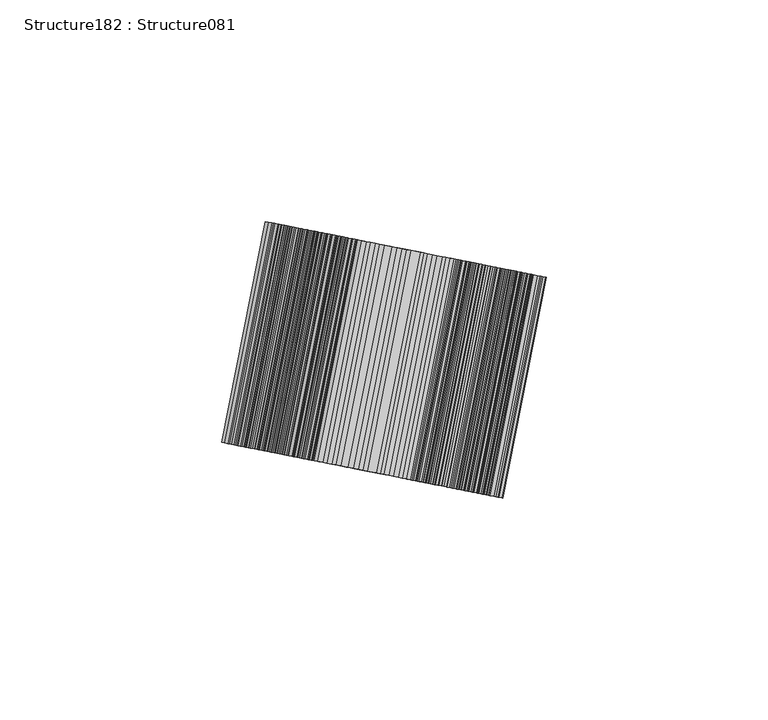
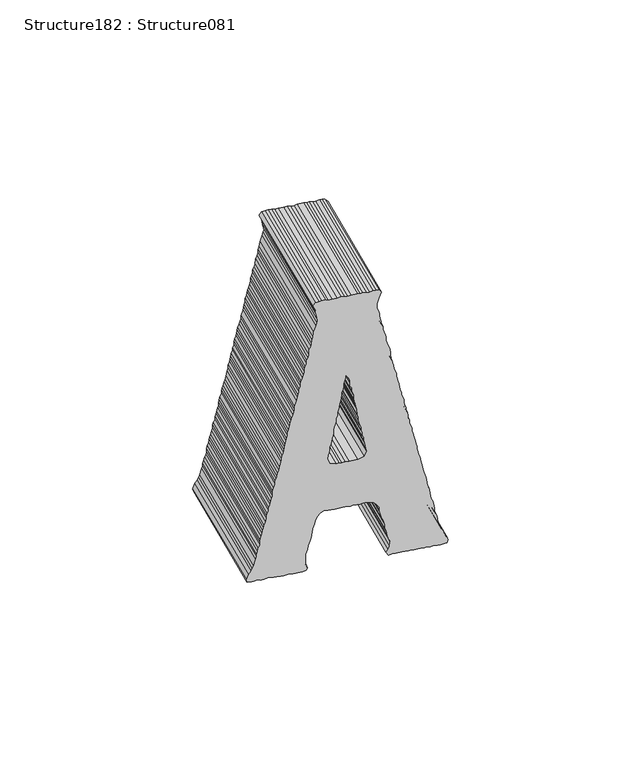
"""IFC4 building model written with IfcOpenShell, lengths in millimetres: proxy geometry, Structure182 : Structure081."""

from ifc_helpers import new_model, si_unit, frame, origin, place, context, project, spatial, polyline, outline, extrude, source, transform, mapped, element, save


def structure182_structure081_149fff3d(model_context):
    return source(origin(), model_context, "Body", "SweptSolid", [
        extrude(outline(polyline([(0.9094651, 0.0), (2.0811665, -0.5212701), (2.9906316, -0.6507871), (4.1562841, -0.780304), (5.1991801, -1.1720571), (5.9748585, -1.3012184), (7.1504738, -1.6890575), (8.1894559, -1.6890575), (9.3551083, -2.0808107), (10.2645735, -2.3398445), (11.4362748, -2.5981668), (12.3453841, -2.8611147), (13.3818755, -2.9902758), (14.1582655, -3.378115), (15.4626861, -3.509411), (16.3721513, -3.509411), (17.5385154, -3.7698682), (19.491944, -4.4188761), (20.2718921, -4.6793333), (21.3101626, -4.9383672), (22.3470097, -4.9383672), (23.2561191, -5.1988244), (24.4278204, -5.5866635), (25.4700048, -5.9766376), (26.6363689, -5.9766376), (27.4124031, -6.3666117), (28.7175354, -6.6274247), (30.535754, -7.0173988), (31.5743802, -7.1483389), (32.7400327, -7.4073728), (33.6555467, -7.7969911), (35.4741211, -7.7969911), (36.5102567, -7.5361781), (37.5492387, -7.275721), (38.3288311, -6.8878819), (39.3671015, -6.3666117), (40.4099976, -7.275721), (40.5395145, -8.1851861), (40.5395145, -9.0964303), (40.2826155, -10.2659967), (40.2826155, -11.3042672), (40.5395145, -12.4745453), (40.4099976, -13.2523586), (40.5395145, -14.1639585), (40.5395145, -16.2429902), (40.2826155, -17.2791257), (40.2826155, -18.3198869), (40.5395145, -19.4915882), (40.4099976, -20.6575964), (40.4099976, -22.3466539), (40.2826155, -23.5183553), (40.5395145, -24.4274646), (40.5395145, -25.595252), (40.4099976, -26.5047171), (40.2826155, -27.6742836), (39.2382962, -28.4545875), (38.3288311, -27.9372314), (37.4197218, -27.6742836), (36.6397736, -27.5454783), (35.4741211, -27.2846653), (33.5199809, -26.8964703), (32.6112274, -27.1576391), (31.4448633, -27.4138264), (29.3636968, -28.1937746), (27.545834, -28.4545875), (26.5089869, -28.7150447), (25.3372855, -28.8445616), (24.2943895, -29.1032397), (23.2561191, -29.6262889), (21.3101626, -29.7540268), (20.2718921, -30.0144839), (19.491944, -30.5336191), (18.3202426, -30.5336191), (17.2816164, -30.9235932), (16.3721513, -31.1840503), (15.3356599, -31.1840503), (14.1582655, -31.4427285), (13.1253323, -31.8330584), (12.2158672, -32.2230324), (11.4362748, -32.3518377), (10.2645735, -32.4834896), (9.3551083, -32.8731078), (8.1894559, -32.8731078), (7.1504738, -33.2613029), (6.2374505, -33.3925989), (5.0714422, -33.653056), (3.2475306, -34.302064), (2.0811665, -34.302064), (1.1720572, -34.5625212), (0.1334309, -34.8208434), (-1.0382704, -35.3421135), (-1.8178628, -35.4716305), (-2.8568449, -35.7303085), (-3.8990293, -35.8616046), (-5.0653934, -36.2515787), (-5.8471206, -36.5099009), (-7.0166871, -36.5099009), (-8.1826954, -36.899875), (-8.9644226, -37.0315268), (-10.1364798, -37.419366), (-11.1690572, -37.5506621), (-12.2115974, -37.680179), (-12.9915456, -37.9406362), (-14.03373, -38.3284753), (-15.3292552, -38.4601271), (-16.3678815, -38.7205843), (-18.1861001, -39.1084235), (-19.3581573, -39.3692365), (-20.2672666, -39.7574314), (-21.4371888, -40.0178886), (-22.2189161, -40.2783458), (-23.1223323, -40.5370239), (-24.1648726, -40.5370239), (-25.465735, -41.0586498), (-26.5025822, -41.316972), (-27.4173846, -41.4464889), (-28.4560108, -41.4464889), (-29.235959, -41.7069461), (-30.5311284, -42.0986993), (-31.3110766, -42.2264372), (-32.3536168, -42.6181903), (-33.5214042, -42.6181903), (-34.4308693, -43.1355464), (-35.3399786, -43.3960036), (-36.37647, -43.3960036), (-37.5424783, -43.6564608), (-38.7202285, -44.0442999), (-39.6236447, -44.3072478), (-40.405372, -44.5659258), (-41.5752942, -44.695087), (-42.6139205, -45.0850611), (-43.7856218, -45.3455183), (-44.8221132, -45.3455183), (-45.7372714, -45.4732561), (-46.6406876, -45.9963053), (-47.812389, -46.2549833), (-48.8510152, -46.5140173), (-49.7601245, -46.5140173), (-50.6731478, -46.9057704), (-52.8777823, -47.5540667), (-53.7929405, -47.941906), (-54.5689747, -48.3340149), (-55.738897, -49.1118282), (-57.5532016, -49.7626152), (-58.4665807, -49.5035814), (-58.5957419, -48.2030748), (-58.4665807, -47.4227707), (-58.3331498, -46.2549833), (-58.5957419, -45.2167129), (-58.5957419, -44.0442999), (-58.3331498, -43.0060295), (-58.3331498, -42.0986993), (-58.4665807, -41.0586498), (-58.4665807, -40.1491846), (-58.5957419, -38.8479664), (-58.5957419, -37.9406362), (-58.4665807, -36.899875), (-58.3331498, -35.7303085), (-58.5957419, -34.8208434), (-58.5957419, -31.8330584), (-58.3331498, -30.6627802), (-57.4297336, -30.1440009), (-56.6480063, -30.5336191), (-55.6115149, -30.7940763), (-53.3972734, -30.7940763), (-52.3586471, -30.7940763), (-51.4495378, -30.5336191), (-50.6731478, -30.1440009), (-49.3683714, -30.0144839), (-48.4592621, -29.7540268), (-47.5497969, -29.3636969), (-46.6406876, -29.1032397), (-45.6038405, -28.8445616), (-43.2661308, -28.5855278), (-41.5752942, -27.9372314), (-40.2762109, -27.6742836), (-38.9767716, -27.0259872), (-38.1950444, -26.116878), (-37.4190102, -24.6864985), (-37.6759092, -23.6478723), (-37.6759092, -21.5688406), (-37.5424783, -20.2694015), (-37.5424783, -17.5420735), (-37.6759092, -16.3700164), (-37.4190102, -15.463042), (-37.5424783, -14.4240599), (-37.6759092, -13.3840104), (-37.5424783, -12.4745453), (-37.4190102, -11.1754619), (-37.6759092, -10.3955138), (-38.0676623, -8.8373964), (-38.8476105, -8.0556692), (-40.2762109, -7.0173988), (-41.4422191, -7.0173988), (-42.6139205, -6.75623), (-44.561656, -6.2388738), (-45.3472973, -5.7179595), (-46.5133056, -5.4592815), (-47.2932538, -5.3283413), (-48.33188, -5.3283413), (-49.3683714, -4.8067153), (-50.4126907, -4.6793333), (-51.4495378, -4.5501722), (-52.3586471, -4.158419), (-53.6595096, -3.7698682), (-55.3489229, -3.897606), (-56.6480063, -4.2875802), (-57.2966585, -4.9383672), (-58.5957419, -4.158419), (-58.4665807, -2.9902758), (-58.3331498, -1.9498705), (-58.3331498, 0.1291611), (-58.4665807, 1.1677874), (-58.4665807, 2.2060577), (-58.3331498, 3.1176577), (-58.4665807, 4.0267671), (-58.4665807, 5.3258505), (-58.3331498, 6.1040195), (-58.4665807, 7.4052379), (-58.3331498, 8.1848303), (-58.5957419, 9.2252356), (-58.3331498, 10.3933787), (-58.5957419, 11.563301), (-58.4665807, 12.4724103), (-58.3331498, 13.5128156), (-58.3331498, 14.5496628), (-57.2966585, 14.941416), (-56.3875492, 14.6809589), (-55.738897, 14.0301718), (-54.5689747, 13.7718495), (-53.7929405, 13.3818755), (-52.6151903, 12.8602495), (-50.6731478, 11.9511402), (-49.8875066, 11.692818), (-48.5941162, 11.563301), (-47.5497969, 11.3028439), (-46.6406876, 11.04381), (-45.8646534, 10.6520569), (-44.5616561, 10.5225398), (-42.6139205, 10.2638618), (-41.4422191, 9.8738878), (-40.5384471, 9.4821345), (-39.6236447, 9.2252356), (-38.4576364, 9.0942954), (-37.4190102, 8.9626435), (-36.5059869, 8.8338382), (-35.6004358, 8.3143472), (-34.2956593, 8.1848303), (-33.3922431, 8.0535342), (-32.3536168, 7.9243731), (-31.4405935, 7.5365339), (-30.4019673, 7.1447807), (-29.235959, 6.8857468), (-27.5447666, 6.6252897), (-26.3752002, 6.2353156), (-25.203143, 6.1040195), (-24.4235506, 5.8474765), (-23.3849244, 5.4553674), (-22.4793732, 5.3258505), (-21.3037579, 4.9362323), (-20.2672666, 4.9362323), (-19.3581573, 4.6750634), (-18.319531, 4.4167412), (-17.1474738, 4.158419), (-15.2018732, 3.636793), (-14.1632469, 3.3777591), (-13.1207067, 3.3777591), (-12.2115974, 2.986006), (-11.3024881, 2.5981668), (-10.0012698, 2.5981668), (-9.2270147, 2.0772524), (-8.1826954, 2.0772524), (-7.0166871, 1.9498704), (-5.9745027, 1.4282444), (-5.0653934, 1.4282444), (-4.1619771, 0.9091093), (-2.8568449, 0.7799482), (-1.9473797, 0.7799482), (-0.7817273, 0.2604572), (0.0, 0.0), (0.9094651, 0.0)]), holes=[polyline([(-20.9137838, -13.9010107), (-20.9137838, -16.8912865), (-20.7903157, -18.0590739), (-21.0472147, -19.231131), (-20.7903157, -20.1398845), (-20.9137838, -21.0493497), (-20.2672666, -22.997441), (-18.5817672, -23.6478723), (-17.2809048, -23.3874152), (-16.3678815, -23.1262464), (-15.4623303, -22.870059), (-14.1632469, -22.997441), (-13.2480888, -22.47795), (-12.2115974, -22.3466539), (-11.3024881, -22.2174928), (-10.393023, -21.8292978), (-9.3508386, -21.6983577), (-8.3122123, -21.6983577), (-7.146204, -21.5688406), (-6.3644768, -21.1806457), (-5.3276296, -20.9201885), (-4.2854452, -20.9201885), (-3.117302, -20.4010534), (-1.9473797, -20.4010534), (-1.0382704, -20.0089444), (-0.2561874, -19.8794274), (1.0389821, -19.7481314), (2.0811665, -19.4915882), (3.1180136, -19.231131), (4.0274787, -19.099835), (5.0714422, -19.099835), (6.1082894, -18.580344), (7.0177545, -18.4508271), (8.1894559, -18.4508271), (9.2216774, -18.0590739), (10.1368356, -17.8025307), (11.0463007, -17.8025307), (10.1368356, -17.1520995), (9.0928721, -16.7617696), (8.056025, -16.6308294), (6.8900167, -16.6308294), (6.1082894, -16.1134732), (4.9365881, -15.9818214), (3.1180136, -15.463042), (1.8189302, -15.333525), (0.9094651, -15.202229), (0.0, -14.9417718), (-1.0382704, -14.8122549), (-2.2078369, -14.4240599), (-4.2854452, -14.292764), (-5.3276296, -14.0323068), (-6.3644768, -13.9010107), (-8.1826954, -13.5128157), (-9.2270147, -12.9936805), (-10.2638619, -12.9936805), (-11.1690572, -12.7332234), (-12.3446725, -12.6037064), (-13.1207067, -12.2115974), (-14.286715, -12.2115974), (-15.4623303, -11.8237582), (-17.2809048, -11.563301), (-18.5817672, -11.3042672), (-20.1377496, -12.0845712), (-20.9137838, -13.9010107)])]), frame((-2036.2341899, 234872.586214, 444.9951864), z_axis=(0.19466222296394123, 0.9808703374813295, 0.0), x_axis=(0.0, 0.0, 1.0)), (0.0, 0.0, 1.0), 50.8),
    ])


if __name__ == "__main__":
    model = new_model("IFC4")
    model_context = context("Model", 3, world=origin())
    ifc_project = project(units=[si_unit("LENGTHUNIT", "METRE", prefix="MILLI")], contexts=[model_context])
    site = spatial("IfcSite", under=ifc_project)
    building = spatial("IfcBuilding", under=site)
    placement = place(None, origin())
    structure182_structure081_shape = structure182_structure081_149fff3d(model_context)
    element("IfcBuildingElementProxy", 1, Name="Structure182 : Structure081", ObjectType="Structure182 : Structure081", at=placement, inside=building, context=model_context, shape_type="MappedRepresentation", body=[
        mapped(structure182_structure081_shape, transform((0.0, 0.0, 0.0), x_axis=(1.0, 0.0, 0.0), y_axis=(0.0, 1.0, 0.0), z_axis=(0.0, 0.0, 1.0))),
    ])
    save(model, "model.ifc")

# Revit data of these elements
# Type "Structure182 : Structure081"
#   NameOverride = "Structure081"
# Element 1 (IfcBuildingElementProxy, "Structure182 : Structure081")
#   Materials on its faces: "BRUSHED ALUMINUM LETTERING"
# Materials
#   "BRUSHED ALUMINUM LETTERING": class "Unassigned", colour RGB 169 181 186, transparency 0, Cost = 0
